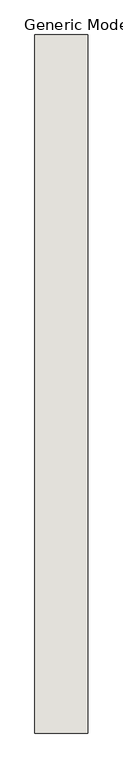
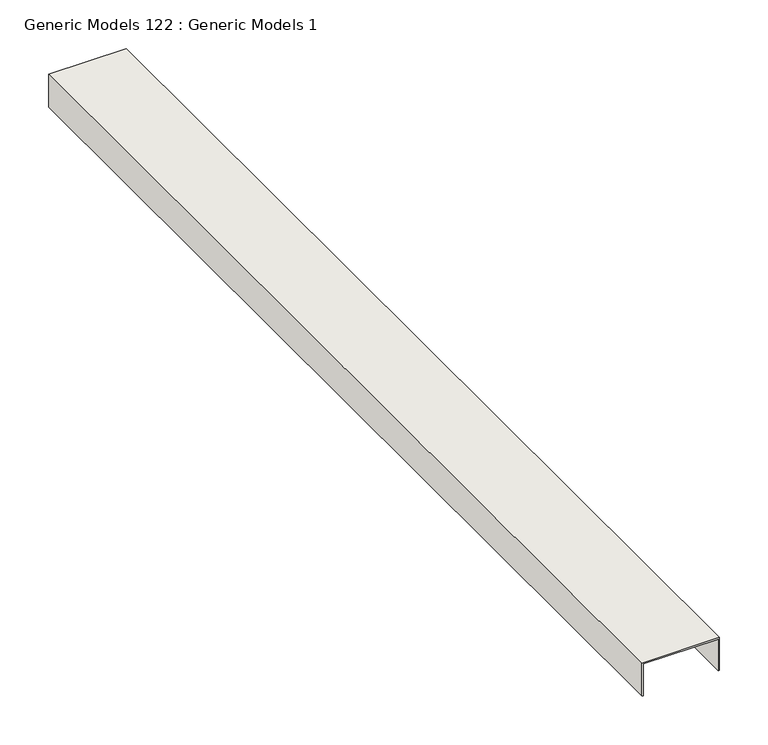
"""IFC4 building model written with IfcOpenShell, lengths in millimetres: wall geometry, Generic Models 122 : Generic Models 1."""

import ifcopenshell
import ifcopenshell.guid

model = None  # the IFC model being written
_history = None  # IfcOwnerHistory: only IFC2X3 demands one
_inside = {}  # id of a spatial element -> (the spatial element, [elements in it])
_under = {}  # id of a project, library or spatial element -> (it, [spatial elements below it])
_declared = {}  # id of a project -> (the project, [libraries it declares])
_typed = {}  # id of a type object -> (the type object, [elements of that type])
_made_of = {}  # id of a material, layer set ... -> (it, [elements and type objects made of it])


def new_model(schema):
    """Start an empty IFC model of exactly this schema.

    Asked for "IFC4X3", IfcOpenShell would pick the latest addendum, in which some entities
    have other attributes; the version numbers below select the first issue.
    IFC2X3 requires an IfcOwnerHistory on every rooted entity: one is made here for all.
    """
    global model, _history
    if schema == "IFC4X3":
        model = ifcopenshell.file(schema_version=(4, 3, 0, 0))
    else:
        model = ifcopenshell.file(schema=schema)
    _inside.clear()
    _under.clear()
    _declared.clear()
    _typed.clear()
    _made_of.clear()
    _history = None
    if model.schema == "IFC2X3":
        org = make("IfcOrganization", Name="unknown")
        user = make(
            "IfcPersonAndOrganization",
            ThePerson=make("IfcPerson", FamilyName="unknown"),
            TheOrganization=org,
        )
        app = make(
            "IfcApplication",
            ApplicationDeveloper=org,
            Version="unknown",
            ApplicationFullName="unknown",
            ApplicationIdentifier="unknown",
        )
        _history = make(
            "IfcOwnerHistory",
            OwningUser=user,
            OwningApplication=app,
            ChangeAction="ADDED",
            CreationDate=0,
        )
    return model


def make(cls, **values):
    """One entity of the class cls with the attributes given. An attribute that is None is left unset."""
    return model.create_entity(
        cls, **{name: value for name, value in values.items() if value is not None}
    )


def rooted(cls, **values):
    """An entity with a GlobalId (a new one), such as an element, a storey or a relation."""
    return make(cls, GlobalId=ifcopenshell.guid.new(), OwnerHistory=_history, **values)


def si_unit(unit_type, name, prefix=None):
    """IfcSIUnit, for example si_unit("LENGTHUNIT", "METRE", prefix="MILLI")."""
    return make("IfcSIUnit", UnitType=unit_type, Prefix=prefix, Name=name)


def assignment(units):
    """IfcUnitAssignment: the units of a project."""
    return None if units is None else make("IfcUnitAssignment", Units=units)


def point(xyz):
    """IfcCartesianPoint."""
    return None if xyz is None else make("IfcCartesianPoint", Coordinates=xyz)


def direction(xyz):
    """IfcDirection."""
    return None if xyz is None else make("IfcDirection", DirectionRatios=xyz)


def frame(location, z_axis=None, x_axis=None):
    """IfcAxis2Placement3D, a coordinate frame: its origin and axes. An axis left out is left unset."""
    return make(
        "IfcAxis2Placement3D",
        Location=point(location),
        Axis=direction(z_axis),
        RefDirection=direction(x_axis),
    )


def origin():
    """The frame at (0, 0, 0) with its axes left unset."""
    return frame((0.0, 0.0, 0.0))


def place(relative_to, where):
    """IfcLocalPlacement: puts the frame where relative to a parent placement (None: the world)."""
    return make(
        "IfcLocalPlacement", PlacementRelTo=relative_to, RelativePlacement=where
    )


def context(
    kind, dimensions, precision=None, world=None, true_north=None, identifier=None
):
    """IfcGeometricRepresentationContext, for example the 3D "Model" context."""
    return make(
        "IfcGeometricRepresentationContext",
        ContextIdentifier=identifier,
        ContextType=kind,
        CoordinateSpaceDimension=dimensions,
        Precision=precision,
        WorldCoordinateSystem=world,
        TrueNorth=true_north,
    )


def project(units=None, contexts=None):
    """IfcProject with its units and contexts."""
    return rooted(
        "IfcProject",
        Name="project",
        RepresentationContexts=contexts,
        UnitsInContext=assignment(units),
    )


def spatial(cls, under=None, at=None, **own):
    """A site, building, storey or space (cls), placed at a placement, below another one or the project."""
    s = rooted(cls, ObjectPlacement=at, **own)
    if under is not None:
        _under.setdefault(under.id(), (under, []))[1].append(s)
    return s


def polyline(points):
    """IfcPolyline through the points."""
    return make("IfcPolyline", Points=[point(p) for p in points])


def outline(outer, holes=None, kind="AREA"):
    """IfcArbitraryClosedProfileDef: a profile drawn as a closed curve; with holes, ...WithVoids."""
    if holes is None:
        return make("IfcArbitraryClosedProfileDef", ProfileType=kind, OuterCurve=outer)
    return make(
        "IfcArbitraryProfileDefWithVoids",
        ProfileType=kind,
        OuterCurve=outer,
        InnerCurves=holes,
    )


def extrude(swept, where, along, depth):
    """IfcExtrudedAreaSolid: the profile swept, set in the frame where, extruded along a direction by depth."""
    return make(
        "IfcExtrudedAreaSolid",
        SweptArea=swept,
        Position=where,
        ExtrudedDirection=direction(along),
        Depth=depth,
    )


def shape(context_of_items, identifier, shape_type, items):
    """IfcShapeRepresentation: the items that make up one representation, for example the "Body"."""
    return make(
        "IfcShapeRepresentation",
        ContextOfItems=context_of_items,
        RepresentationIdentifier=identifier,
        RepresentationType=shape_type,
        Items=items,
    )


def source(mapping_origin, context_of_items, identifier, shape_type, items):
    """IfcRepresentationMap: a shape defined once, which mapped items show again and again."""
    return make(
        "IfcRepresentationMap",
        MappingOrigin=mapping_origin,
        MappedRepresentation=shape(context_of_items, identifier, shape_type, items),
    )


def transform(
    local_origin,
    x_axis=None,
    y_axis=None,
    z_axis=None,
    scale=None,
    scale2=None,
    scale3=None,
    uniform=True,
):
    """IfcCartesianTransformationOperator3D, or its non-uniform kind. x_axis, y_axis, z_axis: its Axis1, 2, 3."""
    if uniform:
        return make(
            "IfcCartesianTransformationOperator3D",
            Axis1=direction(x_axis),
            Axis2=direction(y_axis),
            LocalOrigin=point(local_origin),
            Scale=scale,
            Axis3=direction(z_axis),
        )
    return make(
        "IfcCartesianTransformationOperator3DnonUniform",
        Axis1=direction(x_axis),
        Axis2=direction(y_axis),
        LocalOrigin=point(local_origin),
        Scale=scale,
        Axis3=direction(z_axis),
        Scale2=scale2,
        Scale3=scale3,
    )


def mapped(mapping_source, mapping_target):
    """IfcMappedItem: shows the shape of a source again, moved by a transform."""
    return make(
        "IfcMappedItem", MappingSource=mapping_source, MappingTarget=mapping_target
    )


def made_of(thing, what):
    """Note that an element or type object is made of a material, layer set ...; save() writes the relation."""
    if what is not None:
        _made_of.setdefault(what.id(), (what, []))[1].append(thing)
    return thing


def element(
    cls,
    number,
    at=None,
    inside=None,
    cuts=None,
    type_object=None,
    material=None,
    context=None,
    identifier="Body",
    shape_type=None,
    held_by="IfcProductDefinitionShape",
    body=None,
    shapes=None,
    **own,
):
    """One element of the class cls, such as IfcWall. Its Tag is "e" and its number.

    at: its placement. inside: the storey or other place that contains it. cuts: it is an
    opening in that element (IfcRelVoidsElement). A single representation is given by context,
    identifier, shape_type and body (its items); several are given by shapes. held_by: the class
    of the entity that holds the representations. save() writes the other relations.
    """
    e = rooted(cls, Tag="e%d" % number, ObjectPlacement=at, **own)
    if body is not None:
        shapes = [shape(context, identifier, shape_type, body)]
    if shapes is not None:
        e.Representation = make(held_by, Representations=shapes)
    if inside is not None:
        _inside.setdefault(inside.id(), (inside, []))[1].append(e)
    if cuts is not None:
        rooted(
            "IfcRelVoidsElement", RelatingBuildingElement=cuts, RelatedOpeningElement=e
        )
    if type_object is not None:
        _typed.setdefault(type_object.id(), (type_object, []))[1].append(e)
    return made_of(e, material)


def aggregate(whole, parts):
    """IfcRelAggregates: a whole, such as a stair, and the parts it consists of."""
    return rooted("IfcRelAggregates", RelatingObject=whole, RelatedObjects=parts)


def save(model, path):
    """Write the relations noted so far, then the file.

    IfcRelAggregates (storeys below a building ...), IfcRelContainedInSpatialStructure (elements
    in a storey), IfcRelDefinesByType, IfcRelAssociatesMaterial and IfcRelDeclares: one each for
    every whole, place, type object, material and project.
    """
    for whole, parts in _under.values():
        aggregate(whole, parts)
    for where, things in _inside.values():
        rooted(
            "IfcRelContainedInSpatialStructure",
            RelatedElements=things,
            RelatingStructure=where,
        )
    for kind, things in _typed.values():
        rooted("IfcRelDefinesByType", RelatedObjects=things, RelatingType=kind)
    for what, things in _made_of.values():
        rooted("IfcRelAssociatesMaterial", RelatedObjects=things, RelatingMaterial=what)
    for by, libraries in _declared.values():
        rooted("IfcRelDeclares", RelatingContext=by, RelatedDefinitions=libraries)
    model.write(path)


def generic_models_122_generic_models_1_edb11e6f(model_context):
    return source(origin(), model_context, "Body", "SweptSolid", [
        extrude(outline(polyline([(2457.45, 51003.2), (2457.45, 50911.125), (2416.175, 50911.125), (2416.175, 50912.7125), (2455.8625, 50912.7125), (2455.8625, 51001.6125), (2416.175, 51001.6125), (2416.175, 51003.2), (2457.45, 51003.2)])), frame((0.0, 0.0, 0.0), z_axis=(0.0, 1.0, 0.0), x_axis=(0.0, 0.0, 1.0)), (0.0, 0.0, 1.0), 1219.2),
    ])


if __name__ == "__main__":
    model = new_model("IFC4")
    model_context = context("Model", 3, world=origin())
    ifc_project = project(units=[si_unit("LENGTHUNIT", "METRE", prefix="MILLI")], contexts=[model_context])
    site = spatial("IfcSite", under=ifc_project)
    building = spatial("IfcBuilding", under=site)
    placement = place(None, origin())
    generic_models_122_generic_models_1_shape = generic_models_122_generic_models_1_edb11e6f(model_context)
    element("IfcWall", 1, ObjectType="Generic Models 122 : Generic Models 1", at=placement, inside=building, context=model_context, shape_type="MappedRepresentation", body=[
        mapped(generic_models_122_generic_models_1_shape, transform((0.0, 0.0, 0.0), x_axis=(1.0, 0.0, 0.0), y_axis=(0.0, 1.0, 0.0), z_axis=(0.0, 0.0, 1.0))),
    ])
    save(model, "model.ifc")

# Revit data of these elements
# Element 1 (IfcWall, "Generic Models 122 : Generic Models 1")
#   Materials on its faces: "DEEP LEG OF DEFLECTION TRACK (2\" MIN. DEFLECTION)"
# Materials
#   "DEEP LEG OF DEFLECTION TRACK (2\" MIN. DEFLECTION)": class "Unassigned", colour RGB 210 209 208, transparency 0, Keynote = "M05121300.02", Cost = 0
